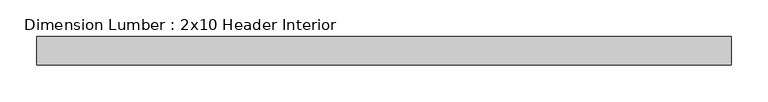
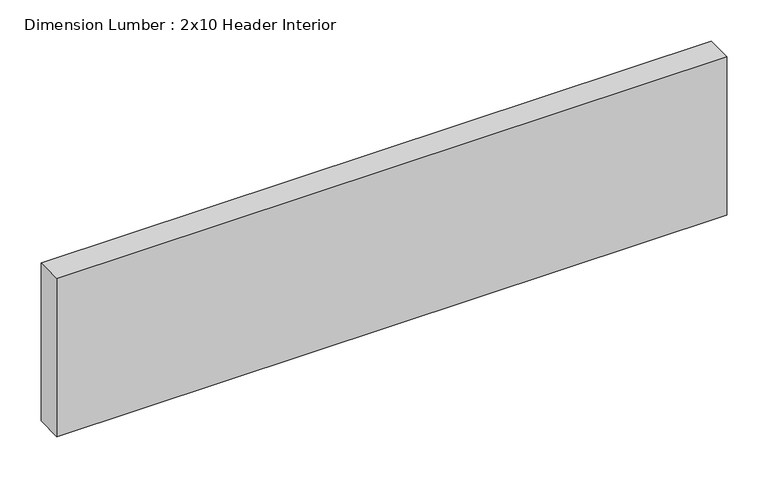
"""IFC4 building model written with IfcOpenShell, lengths in millimetres: beam geometry, Dimension Lumber : 2x10 Header Interior."""

from ifc_helpers import new_model, si_unit, frame, origin, place, context, project, spatial, polyline, outline, extrude, source, transform, mapped, element, save


def dimension_lumber_2x10_header_interior_e412fa49(model_context):
    return source(origin(), model_context, "Body", "SweptSolid", [
        extrude(outline(polyline([(468.709375, 19.05), (468.709375, -19.05), (-471.090625, -19.05), (-471.090625, 19.05), (468.709375, 19.05)])), frame((0.0, 0.0, -117.475), z_axis=(0.0, 0.0, 1.0), x_axis=(1.0, 0.0, 0.0)), (0.0, 0.0, 1.0), 234.95),
    ])


if __name__ == "__main__":
    model = new_model("IFC4")
    model_context = context("Model", 3, world=origin())
    ifc_project = project(units=[si_unit("LENGTHUNIT", "METRE", prefix="MILLI")], contexts=[model_context])
    site = spatial("IfcSite", under=ifc_project)
    building = spatial("IfcBuilding", under=site)
    placement = place(None, origin())
    dimension_lumber_2x10_header_interior_shape = dimension_lumber_2x10_header_interior_e412fa49(model_context)
    element("IfcBeam", 1, ObjectType="Dimension Lumber : 2x10 Header Interior", at=placement, inside=building, context=model_context, shape_type="MappedRepresentation", body=[
        mapped(dimension_lumber_2x10_header_interior_shape, transform((0.0, 0.0, 0.0), x_axis=(1.0, 0.0, 0.0), y_axis=(0.0, 1.0, 0.0), z_axis=(0.0, 0.0, 1.0))),
    ])
    save(model, "model.ifc")

# Revit data of these elements
# Type "Dimension Lumber : 2x10 Header Interior"
#   Assembly Code = "B10"
#   A = 0.0963889 SF
#   Length [instance default] = 5' - 0"
#   b = 0' - 1 1/2"
#   d = 0' - 9 1/4"
#   Structural Material [instance default] = Softwood, Lumber
# Element 1 (IfcBeam, "Dimension Lumber : 2x10 Header Interior")
#   Structural Material = Douglas Fir #2
#   Materials on its faces: "Douglas Fir #2"
# Materials
#   "Softwood, Lumber": class "Wood", colour RGB 223 192 134, transparency 0, Description = "Pinus Echinata", Cost = 0
#   "Douglas Fir #2": class "Wood", colour RGB 223 192 134, transparency 0, Description = "Pinus Echinata", Cost = 0
